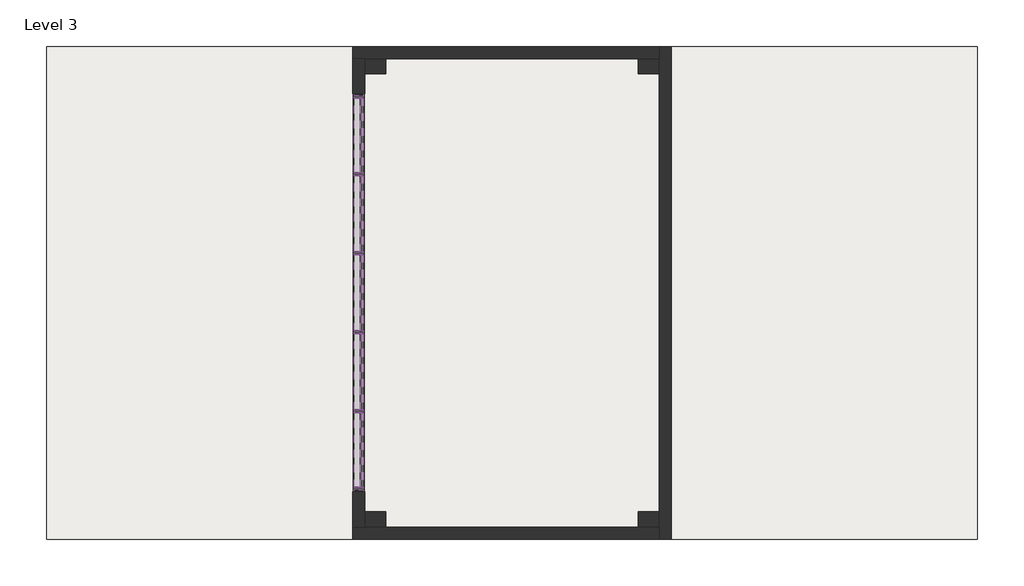
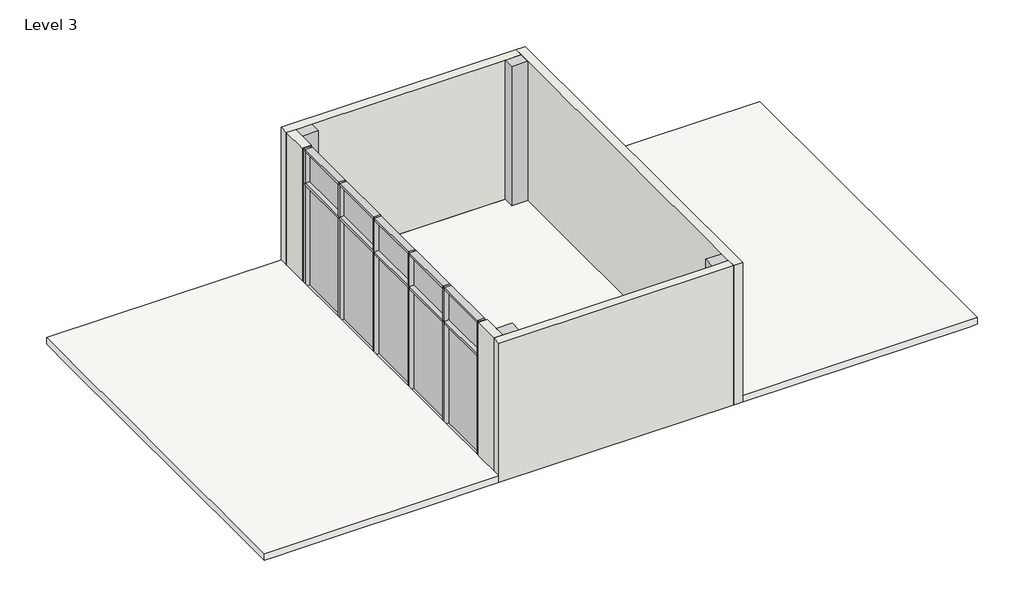
# One storey: 27 members, 10 plates, 5 walls, 4 columns, 2 roofs, 1 slab.
"""IFC4 building model written with IfcOpenShell, lengths in millimetres."""

import ifcopenshell
import ifcopenshell.guid

model = None  # the IFC model being written
_history = None  # IfcOwnerHistory: only IFC2X3 demands one
_inside = {}  # id of a spatial element -> (the spatial element, [elements in it])
_under = {}  # id of a project, library or spatial element -> (it, [spatial elements below it])
_declared = {}  # id of a project -> (the project, [libraries it declares])
_typed = {}  # id of a type object -> (the type object, [elements of that type])
_made_of = {}  # id of a material, layer set ... -> (it, [elements and type objects made of it])


def new_model(schema):
    """Start an empty IFC model of exactly this schema.

    Asked for "IFC4X3", IfcOpenShell would pick the latest addendum, in which some entities
    have other attributes; the version numbers below select the first issue.
    IFC2X3 requires an IfcOwnerHistory on every rooted entity: one is made here for all.
    """
    global model, _history
    if schema == "IFC4X3":
        model = ifcopenshell.file(schema_version=(4, 3, 0, 0))
    else:
        model = ifcopenshell.file(schema=schema)
    _inside.clear()
    _under.clear()
    _declared.clear()
    _typed.clear()
    _made_of.clear()
    _history = None
    if model.schema == "IFC2X3":
        org = make("IfcOrganization", Name="unknown")
        user = make(
            "IfcPersonAndOrganization",
            ThePerson=make("IfcPerson", FamilyName="unknown"),
            TheOrganization=org,
        )
        app = make(
            "IfcApplication",
            ApplicationDeveloper=org,
            Version="unknown",
            ApplicationFullName="unknown",
            ApplicationIdentifier="unknown",
        )
        _history = make(
            "IfcOwnerHistory",
            OwningUser=user,
            OwningApplication=app,
            ChangeAction="ADDED",
            CreationDate=0,
        )
    return model


def make(cls, **values):
    """One entity of the class cls with the attributes given. An attribute that is None is left unset."""
    return model.create_entity(
        cls, **{name: value for name, value in values.items() if value is not None}
    )


def rooted(cls, **values):
    """An entity with a GlobalId (a new one), such as an element, a storey or a relation."""
    return make(cls, GlobalId=ifcopenshell.guid.new(), OwnerHistory=_history, **values)


def si_unit(unit_type, name, prefix=None):
    """IfcSIUnit, for example si_unit("LENGTHUNIT", "METRE", prefix="MILLI")."""
    return make("IfcSIUnit", UnitType=unit_type, Prefix=prefix, Name=name)


def assignment(units):
    """IfcUnitAssignment: the units of a project."""
    return None if units is None else make("IfcUnitAssignment", Units=units)


def point(xyz):
    """IfcCartesianPoint."""
    return None if xyz is None else make("IfcCartesianPoint", Coordinates=xyz)


def direction(xyz):
    """IfcDirection."""
    return None if xyz is None else make("IfcDirection", DirectionRatios=xyz)


def frame(location, z_axis=None, x_axis=None):
    """IfcAxis2Placement3D, a coordinate frame: its origin and axes. An axis left out is left unset."""
    return make(
        "IfcAxis2Placement3D",
        Location=point(location),
        Axis=direction(z_axis),
        RefDirection=direction(x_axis),
    )


def origin():
    """The frame at (0, 0, 0) with its axes left unset."""
    return frame((0.0, 0.0, 0.0))


def origin_with_axes():
    """The frame at (0, 0, 0) with the z axis (0, 0, 1) and the x axis (1, 0, 0) written out."""
    return frame((0.0, 0.0, 0.0), z_axis=(0.0, 0.0, 1.0), x_axis=(1.0, 0.0, 0.0))


def place(relative_to, where):
    """IfcLocalPlacement: puts the frame where relative to a parent placement (None: the world)."""
    return make(
        "IfcLocalPlacement", PlacementRelTo=relative_to, RelativePlacement=where
    )


def context(
    kind, dimensions, precision=None, world=None, true_north=None, identifier=None
):
    """IfcGeometricRepresentationContext, for example the 3D "Model" context."""
    return make(
        "IfcGeometricRepresentationContext",
        ContextIdentifier=identifier,
        ContextType=kind,
        CoordinateSpaceDimension=dimensions,
        Precision=precision,
        WorldCoordinateSystem=world,
        TrueNorth=true_north,
    )


def project(units=None, contexts=None):
    """IfcProject with its units and contexts."""
    return rooted(
        "IfcProject",
        Name="project",
        RepresentationContexts=contexts,
        UnitsInContext=assignment(units),
    )


def spatial(cls, under=None, at=None, **own):
    """A site, building, storey or space (cls), placed at a placement, below another one or the project."""
    s = rooted(cls, ObjectPlacement=at, **own)
    if under is not None:
        _under.setdefault(under.id(), (under, []))[1].append(s)
    return s


def polyline(points):
    """IfcPolyline through the points."""
    return make("IfcPolyline", Points=[point(p) for p in points])


def outline(outer, holes=None, kind="AREA"):
    """IfcArbitraryClosedProfileDef: a profile drawn as a closed curve; with holes, ...WithVoids."""
    if holes is None:
        return make("IfcArbitraryClosedProfileDef", ProfileType=kind, OuterCurve=outer)
    return make(
        "IfcArbitraryProfileDefWithVoids",
        ProfileType=kind,
        OuterCurve=outer,
        InnerCurves=holes,
    )


def extrude(swept, where, along, depth):
    """IfcExtrudedAreaSolid: the profile swept, set in the frame where, extruded along a direction by depth."""
    return make(
        "IfcExtrudedAreaSolid",
        SweptArea=swept,
        Position=where,
        ExtrudedDirection=direction(along),
        Depth=depth,
    )


def faces_of(points, faces, orient=None, outer=None):
    """IfcFace entities. A face is a list of loops; a loop is a list of indices into points, from 0.

    orient and outer hold one flag for each loop. By default every Orientation is true, the
    first loop of a face is its IfcFaceOuterBound and the others are IfcFaceBound.
    """
    made = []
    for i, loops in enumerate(faces):
        bounds = []
        for j, loop in enumerate(loops):
            is_outer = j == 0 if outer is None else outer[i][j]
            bounds.append(
                make(
                    "IfcFaceOuterBound" if is_outer else "IfcFaceBound",
                    Bound=make("IfcPolyLoop", Polygon=[points[k] for k in loop]),
                    Orientation=True if orient is None else orient[i][j],
                )
            )
        made.append(make("IfcFace", Bounds=bounds))
    return made


def faceted_brep(points, faces, orient=None, outer=None, voids=None):
    """IfcFacetedBrep: a solid bounded by flat faces; with voids (closed shells), ...WithVoids."""
    shared = [point(p) for p in points]
    hull = make("IfcClosedShell", CfsFaces=faces_of(shared, faces, orient, outer))
    if voids is None:
        return make("IfcFacetedBrep", Outer=hull)
    return make(
        "IfcFacetedBrepWithVoids",
        Outer=hull,
        Voids=[
            make(cls, CfsFaces=faces_of(shared, fs, o, b)) for cls, fs, o, b in voids
        ],
    )


def shape(context_of_items, identifier, shape_type, items):
    """IfcShapeRepresentation: the items that make up one representation, for example the "Body"."""
    return make(
        "IfcShapeRepresentation",
        ContextOfItems=context_of_items,
        RepresentationIdentifier=identifier,
        RepresentationType=shape_type,
        Items=items,
    )


def source(mapping_origin, context_of_items, identifier, shape_type, items):
    """IfcRepresentationMap: a shape defined once, which mapped items show again and again."""
    return make(
        "IfcRepresentationMap",
        MappingOrigin=mapping_origin,
        MappedRepresentation=shape(context_of_items, identifier, shape_type, items),
    )


def transform(
    local_origin,
    x_axis=None,
    y_axis=None,
    z_axis=None,
    scale=None,
    scale2=None,
    scale3=None,
    uniform=True,
):
    """IfcCartesianTransformationOperator3D, or its non-uniform kind. x_axis, y_axis, z_axis: its Axis1, 2, 3."""
    if uniform:
        return make(
            "IfcCartesianTransformationOperator3D",
            Axis1=direction(x_axis),
            Axis2=direction(y_axis),
            LocalOrigin=point(local_origin),
            Scale=scale,
            Axis3=direction(z_axis),
        )
    return make(
        "IfcCartesianTransformationOperator3DnonUniform",
        Axis1=direction(x_axis),
        Axis2=direction(y_axis),
        LocalOrigin=point(local_origin),
        Scale=scale,
        Axis3=direction(z_axis),
        Scale2=scale2,
        Scale3=scale3,
    )


def mapped(mapping_source, mapping_target):
    """IfcMappedItem: shows the shape of a source again, moved by a transform."""
    return make(
        "IfcMappedItem", MappingSource=mapping_source, MappingTarget=mapping_target
    )


def made_of(thing, what):
    """Note that an element or type object is made of a material, layer set ...; save() writes the relation."""
    if what is not None:
        _made_of.setdefault(what.id(), (what, []))[1].append(thing)
    return thing


def element(
    cls,
    number,
    at=None,
    inside=None,
    cuts=None,
    type_object=None,
    material=None,
    context=None,
    identifier="Body",
    shape_type=None,
    held_by="IfcProductDefinitionShape",
    body=None,
    shapes=None,
    **own,
):
    """One element of the class cls, such as IfcWall. Its Tag is "e" and its number.

    at: its placement. inside: the storey or other place that contains it. cuts: it is an
    opening in that element (IfcRelVoidsElement). A single representation is given by context,
    identifier, shape_type and body (its items); several are given by shapes. held_by: the class
    of the entity that holds the representations. save() writes the other relations.
    """
    e = rooted(cls, Tag="e%d" % number, ObjectPlacement=at, **own)
    if body is not None:
        shapes = [shape(context, identifier, shape_type, body)]
    if shapes is not None:
        e.Representation = make(held_by, Representations=shapes)
    if inside is not None:
        _inside.setdefault(inside.id(), (inside, []))[1].append(e)
    if cuts is not None:
        rooted(
            "IfcRelVoidsElement", RelatingBuildingElement=cuts, RelatedOpeningElement=e
        )
    if type_object is not None:
        _typed.setdefault(type_object.id(), (type_object, []))[1].append(e)
    return made_of(e, material)


def aggregate(whole, parts):
    """IfcRelAggregates: a whole, such as a stair, and the parts it consists of."""
    return rooted("IfcRelAggregates", RelatingObject=whole, RelatedObjects=parts)


def save(model, path):
    """Write the relations noted so far, then the file.

    IfcRelAggregates (storeys below a building ...), IfcRelContainedInSpatialStructure (elements
    in a storey), IfcRelDefinesByType, IfcRelAssociatesMaterial and IfcRelDeclares: one each for
    every whole, place, type object, material and project.
    """
    for whole, parts in _under.values():
        aggregate(whole, parts)
    for where, things in _inside.values():
        rooted(
            "IfcRelContainedInSpatialStructure",
            RelatedElements=things,
            RelatingStructure=where,
        )
    for kind, things in _typed.values():
        rooted("IfcRelDefinesByType", RelatedObjects=things, RelatingType=kind)
    for what, things in _made_of.values():
        rooted("IfcRelAssociatesMaterial", RelatedObjects=things, RelatingMaterial=what)
    for by, libraries in _declared.values():
        rooted("IfcRelDeclares", RelatingContext=by, RelatedDefinitions=libraries)
    model.write(path)


def rectangular_mullion_50_x_150mm_49395e3f(model_context):
    return source(origin(), model_context, "Body", "SweptSolid", [
        extrude(outline(polyline([(0.0, 75.0), (0.0, -75.0), (-50.0, -75.0), (-50.0, 75.0), (0.0, 75.0)])), frame((0.0, 0.0, -1240.0000002), z_axis=(0.0, 0.0, 1.0), x_axis=(1.0, 0.0, 0.0)), (0.0, 0.0, 1.0), 1240.0000002),
    ])


def rectangular_mullion_50_x_150mm_673792d4(model_context):
    return source(origin(), model_context, "Body", "SweptSolid", [
        extrude(outline(polyline([(0.0, 75.0), (0.0, -75.0), (-50.0, -75.0), (-50.0, 75.0), (0.0, 75.0)])), frame((0.0, 0.0, -1264.9999999), z_axis=(0.0, 0.0, 1.0), x_axis=(1.0, 0.0, 0.0)), (0.0, 0.0, 1.0), 1264.9999999),
    ])


def rectangular_mullion_50_x_150mm_23e890aa(model_context):
    return source(origin(), model_context, "Body", "SweptSolid", [
        extrude(outline(polyline([(25.0, 75.0), (25.0, -75.0), (-25.0, -75.0), (-25.0, 75.0), (25.0, 75.0)])), frame((0.0, 0.0, -1240.0000002), z_axis=(0.0, 0.0, 1.0), x_axis=(1.0, 0.0, 0.0)), (0.0, 0.0, 1.0), 1240.0000002),
    ])


def rectangular_mullion_50_x_150mm_97c2790d(model_context):
    return source(origin(), model_context, "Body", "SweptSolid", [
        extrude(outline(polyline([(25.0, 75.0), (25.0, -75.0), (-25.0, -75.0), (-25.0, 75.0), (25.0, 75.0)])), frame((0.0, 0.0, -1264.9999999), z_axis=(0.0, 0.0, 1.0), x_axis=(1.0, 0.0, 0.0)), (0.0, 0.0, 1.0), 1264.9999999),
    ])


def rectangular_mullion_50_x_150mm_6225e4e3(model_context):
    return source(origin(), model_context, "Body", "SweptSolid", [
        extrude(outline(polyline([(25.0, 75.0), (25.0, -75.0), (-25.0, -75.0), (-25.0, 75.0), (25.0, 75.0)])), frame((0.0, 0.0, -2400.0), z_axis=(0.0, 0.0, 1.0), x_axis=(1.0, 0.0, 0.0)), (0.0, 0.0, 1.0), 2400.0),
    ])


def rectangular_mullion_50_x_150mm_14f10ac7(model_context):
    return source(origin(), model_context, "Body", "SweptSolid", [
        extrude(outline(polyline([(25.0, 75.0), (25.0, -75.0), (-25.0, -75.0), (-25.0, 75.0), (25.0, 75.0)])), frame((0.0, 0.0, -800.0), z_axis=(0.0, 0.0, 1.0), x_axis=(1.0, 0.0, 0.0)), (0.0, 0.0, 1.0), 800.0),
    ])


def rectangular_mullion_50_x_150mm_662c37b1(model_context):
    return source(origin(), model_context, "Body", "SweptSolid", [
        extrude(outline(polyline([(0.0, 75.0), (0.0, -75.0), (-50.0, -75.0), (-50.0, 75.0), (0.0, 75.0)])), frame((0.0, 0.0, -2400.0), z_axis=(0.0, 0.0, 1.0), x_axis=(1.0, 0.0, 0.0)), (0.0, 0.0, 1.0), 2400.0),
    ])


def rectangular_mullion_50_x_150mm_6ffebc0f(model_context):
    return source(origin(), model_context, "Body", "SweptSolid", [
        extrude(outline(polyline([(0.0, 75.0), (0.0, -75.0), (-50.0, -75.0), (-50.0, 75.0), (0.0, 75.0)])), frame((0.0, 0.0, -800.0), z_axis=(0.0, 0.0, 1.0), x_axis=(1.0, 0.0, 0.0)), (0.0, 0.0, 1.0), 800.0),
    ])


def system_panel_glazed_da598795(model_context):
    return source(origin(), model_context, "Body", "SweptSolid", [
        extrude(outline(polyline([(620.0000001, 24.5), (-620.0000001, 24.5), (-620.0000001, 49.5), (620.0000001, 49.5), (620.0000001, 24.5)])), origin_with_axes(), (0.0, 0.0, 1.0), 2325.0),
    ])


def system_panel_glazed_e4649fa4(model_context):
    return source(origin(), model_context, "Body", "SweptSolid", [
        extrude(outline(polyline([(632.4999999, 24.5), (-632.4999999, 24.5), (-632.4999999, 49.5), (632.4999999, 49.5), (632.4999999, 24.5)])), origin_with_axes(), (0.0, 0.0, 1.0), 2325.0),
    ])


def system_panel_glazed_8692f37a(model_context):
    return source(origin(), model_context, "Body", "SweptSolid", [
        extrude(outline(polyline([(620.0000001, 24.5), (-620.0000001, 24.5), (-620.0000001, 49.5), (620.0000001, 49.5), (620.0000001, 24.5)])), origin_with_axes(), (0.0, 0.0, 1.0), 725.0),
    ])


def system_panel_glazed_8e5047c4(model_context):
    return source(origin(), model_context, "Body", "SweptSolid", [
        extrude(outline(polyline([(632.4999999, 24.5), (-632.4999999, 24.5), (-632.4999999, 49.5), (632.4999999, 49.5), (632.4999999, 24.5)])), origin_with_axes(), (0.0, 0.0, 1.0), 725.0),
    ])


model = new_model("IFC4")

# Units and contexts
model_context = context("Model", 3, world=origin())
ifc_project = project(units=[si_unit("LENGTHUNIT", "METRE", prefix="MILLI")], contexts=[model_context])

# Site, building, storey
site = spatial("IfcSite", under=ifc_project)
building = spatial("IfcBuilding", under=site)
storey = spatial("IfcBuildingStorey", under=building, Name="Level 3", Elevation=6400.0)

# Columns
placement = place(None, origin())
element("IfcColumn", 1, ObjectType="M_Rectangular Column : 350 X 250", at=placement, inside=storey, context=model_context, shape_type="SweptSolid", body=[
    extrude(outline(polyline([(-376.1618676, 3056.2894154), (-26.1618676, 3056.2894154), (-26.1618676, 2806.2894154), (-376.1618676, 2806.2894154), (-376.1618676, 3056.2894154)])), frame((0.0, 0.0, 6400.0), z_axis=(0.0, 0.0, 1.0), x_axis=(1.0, 0.0, 0.0)), (0.0, 0.0, 1.0), 3200.0),
])
element("IfcColumn", 2, ObjectType="M_Rectangular Column : 350 X 250", at=placement, inside=storey, context=model_context, shape_type="SweptSolid", body=[
    extrude(outline(polyline([(-376.1618676, 10606.2894154), (-26.1618676, 10606.2894154), (-26.1618676, 10356.2894154), (-376.1618676, 10356.2894154), (-376.1618676, 10606.2894154)])), frame((0.0, 0.0, 6400.0), z_axis=(0.0, 0.0, 1.0), x_axis=(1.0, 0.0, 0.0)), (0.0, 0.0, 1.0), 3200.0),
])
element("IfcColumn", 3, ObjectType="M_Rectangular Column : 350 X 250", at=placement, inside=storey, context=model_context, shape_type="SweptSolid", body=[
    extrude(outline(polyline([(-4926.1618676, 10606.2894154), (-4576.1618676, 10606.2894154), (-4576.1618676, 10356.2894154), (-4926.1618676, 10356.2894154), (-4926.1618676, 10606.2894154)])), frame((0.0, 0.0, 6400.0), z_axis=(0.0, 0.0, 1.0), x_axis=(1.0, 0.0, 0.0)), (0.0, 0.0, 1.0), 3200.0),
])
element("IfcColumn", 4, ObjectType="M_Rectangular Column : 350 X 250", at=placement, inside=storey, context=model_context, shape_type="SweptSolid", body=[
    extrude(outline(polyline([(-4926.1618676, 3056.2894154), (-4576.1618676, 3056.2894154), (-4576.1618676, 2806.2894154), (-4926.1618676, 2806.2894154), (-4926.1618676, 3056.2894154)])), frame((0.0, 0.0, 6400.0), z_axis=(0.0, 0.0, 1.0), x_axis=(1.0, 0.0, 0.0)), (0.0, 0.0, 1.0), 3200.0),
])

# Members
rectangular_mullion_50_x_150mm_shape = rectangular_mullion_50_x_150mm_49395e3f(model_context)
element("IfcMember", 5, ObjectType="Rectangular Mullion : 50 x 150mm", at=placement, inside=storey, context=model_context, shape_type="MappedRepresentation", body=[
    mapped(rectangular_mullion_50_x_150mm_shape, transform((-5026.1618676, 3468.7894154, 9600.0), x_axis=(0.0, 0.0, 1.0), y_axis=(-1.0, 0.0, 0.0), z_axis=(0.0, -1.0, 0.0))),
])
element("IfcMember", 6, ObjectType="Rectangular Mullion : 50 x 150mm", at=placement, inside=storey, context=model_context, shape_type="MappedRepresentation", body=[
    mapped(rectangular_mullion_50_x_150mm_shape, transform((-5026.1618676, 8703.7894152, 9600.0), x_axis=(0.0, 0.0, 1.0), y_axis=(-1.0, 0.0, 0.0), z_axis=(0.0, -1.0, 0.0))),
])
element("IfcMember", 7, ObjectType="Rectangular Mullion : 50 x 150mm", at=placement, inside=storey, context=model_context, shape_type="MappedRepresentation", body=[
    mapped(rectangular_mullion_50_x_150mm_shape, transform((-5026.1618676, 9943.7894154, 6400.0), x_axis=(0.0, 0.0, -1.0), y_axis=(-1.0, 0.0, 0.0), z_axis=(0.0, 1.0, 0.0))),
])
element("IfcMember", 8, ObjectType="Rectangular Mullion : 50 x 150mm", at=placement, inside=storey, context=model_context, shape_type="MappedRepresentation", body=[
    mapped(rectangular_mullion_50_x_150mm_shape, transform((-5026.1618676, 4708.7894156, 6400.0), x_axis=(0.0, 0.0, -1.0), y_axis=(-1.0, 0.0, 0.0), z_axis=(0.0, 1.0, 0.0))),
])
rectangular_mullion_50_x_150mm_2_shape = rectangular_mullion_50_x_150mm_673792d4(model_context)
element("IfcMember", 9, ObjectType="Rectangular Mullion : 50 x 150mm", at=placement, inside=storey, context=model_context, shape_type="MappedRepresentation", body=[
    mapped(rectangular_mullion_50_x_150mm_2_shape, transform((-5026.1618676, 7388.7894153, 9600.0), x_axis=(0.0, 0.0, 1.0), y_axis=(-1.0, 0.0, 0.0), z_axis=(0.0, -1.0, 0.0))),
])
element("IfcMember", 10, ObjectType="Rectangular Mullion : 50 x 150mm", at=placement, inside=storey, context=model_context, shape_type="MappedRepresentation", body=[
    mapped(rectangular_mullion_50_x_150mm_2_shape, transform((-5026.1618676, 6073.7894154, 9600.0), x_axis=(0.0, 0.0, 1.0), y_axis=(-1.0, 0.0, 0.0), z_axis=(0.0, -1.0, 0.0))),
])
element("IfcMember", 11, ObjectType="Rectangular Mullion : 50 x 150mm", at=placement, inside=storey, context=model_context, shape_type="MappedRepresentation", body=[
    mapped(rectangular_mullion_50_x_150mm_2_shape, transform((-5026.1618676, 4758.7894156, 9600.0), x_axis=(0.0, 0.0, 1.0), y_axis=(-1.0, 0.0, 0.0), z_axis=(0.0, -1.0, 0.0))),
])
element("IfcMember", 12, ObjectType="Rectangular Mullion : 50 x 150mm", at=placement, inside=storey, context=model_context, shape_type="MappedRepresentation", body=[
    mapped(rectangular_mullion_50_x_150mm_2_shape, transform((-5026.1618676, 8653.7894152, 6400.0), x_axis=(0.0, 0.0, -1.0), y_axis=(-1.0, 0.0, 0.0), z_axis=(0.0, 1.0, 0.0))),
])
element("IfcMember", 13, ObjectType="Rectangular Mullion : 50 x 150mm", at=placement, inside=storey, context=model_context, shape_type="MappedRepresentation", body=[
    mapped(rectangular_mullion_50_x_150mm_2_shape, transform((-5026.1618676, 7338.7894153, 6400.0), x_axis=(0.0, 0.0, -1.0), y_axis=(-1.0, 0.0, 0.0), z_axis=(0.0, 1.0, 0.0))),
])
element("IfcMember", 14, ObjectType="Rectangular Mullion : 50 x 150mm", at=placement, inside=storey, context=model_context, shape_type="MappedRepresentation", body=[
    mapped(rectangular_mullion_50_x_150mm_2_shape, transform((-5026.1618676, 6023.7894154, 6400.0), x_axis=(0.0, 0.0, -1.0), y_axis=(-1.0, 0.0, 0.0), z_axis=(0.0, 1.0, 0.0))),
])
rectangular_mullion_50_x_150mm_3_shape = rectangular_mullion_50_x_150mm_23e890aa(model_context)
element("IfcMember", 15, ObjectType="Rectangular Mullion : 50 x 150mm", at=placement, inside=storey, context=model_context, shape_type="MappedRepresentation", body=[
    mapped(rectangular_mullion_50_x_150mm_3_shape, transform((-5026.1618676, 8703.7894152, 8800.0), x_axis=(0.0, 0.0, 1.0), y_axis=(-1.0, 0.0, 0.0), z_axis=(0.0, -1.0, 0.0))),
])
element("IfcMember", 16, ObjectType="Rectangular Mullion : 50 x 150mm", at=placement, inside=storey, context=model_context, shape_type="MappedRepresentation", body=[
    mapped(rectangular_mullion_50_x_150mm_3_shape, transform((-5026.1618676, 3468.7894154, 8800.0), x_axis=(0.0, 0.0, 1.0), y_axis=(-1.0, 0.0, 0.0), z_axis=(0.0, -1.0, 0.0))),
])
rectangular_mullion_50_x_150mm_4_shape = rectangular_mullion_50_x_150mm_97c2790d(model_context)
element("IfcMember", 17, ObjectType="Rectangular Mullion : 50 x 150mm", at=placement, inside=storey, context=model_context, shape_type="MappedRepresentation", body=[
    mapped(rectangular_mullion_50_x_150mm_4_shape, transform((-5026.1618676, 7388.7894153, 8800.0), x_axis=(0.0, 0.0, 1.0), y_axis=(-1.0, 0.0, 0.0), z_axis=(0.0, -1.0, 0.0))),
])
element("IfcMember", 18, ObjectType="Rectangular Mullion : 50 x 150mm", at=placement, inside=storey, context=model_context, shape_type="MappedRepresentation", body=[
    mapped(rectangular_mullion_50_x_150mm_4_shape, transform((-5026.1618676, 6073.7894154, 8800.0), x_axis=(0.0, 0.0, 1.0), y_axis=(-1.0, 0.0, 0.0), z_axis=(0.0, -1.0, 0.0))),
])
element("IfcMember", 19, ObjectType="Rectangular Mullion : 50 x 150mm", at=placement, inside=storey, context=model_context, shape_type="MappedRepresentation", body=[
    mapped(rectangular_mullion_50_x_150mm_4_shape, transform((-5026.1618676, 4758.7894156, 8800.0), x_axis=(0.0, 0.0, 1.0), y_axis=(-1.0, 0.0, 0.0), z_axis=(0.0, -1.0, 0.0))),
])
rectangular_mullion_50_x_150mm_5_shape = rectangular_mullion_50_x_150mm_6225e4e3(model_context)
element("IfcMember", 20, ObjectType="Rectangular Mullion : 50 x 150mm", at=placement, inside=storey, context=model_context, shape_type="MappedRepresentation", body=[
    mapped(rectangular_mullion_50_x_150mm_5_shape, transform((-5026.1618676, 8678.7894152, 6400.0), x_axis=(0.0, -1.0, 0.0), y_axis=(-1.0, 0.0, 0.0), z_axis=(0.0, 0.0, -1.0))),
])
element("IfcMember", 21, ObjectType="Rectangular Mullion : 50 x 150mm", at=placement, inside=storey, context=model_context, shape_type="MappedRepresentation", body=[
    mapped(rectangular_mullion_50_x_150mm_5_shape, transform((-5026.1618676, 7363.7894153, 6400.0), x_axis=(0.0, -1.0, 0.0), y_axis=(-1.0, 0.0, 0.0), z_axis=(0.0, 0.0, -1.0))),
])
element("IfcMember", 22, ObjectType="Rectangular Mullion : 50 x 150mm", at=placement, inside=storey, context=model_context, shape_type="MappedRepresentation", body=[
    mapped(rectangular_mullion_50_x_150mm_5_shape, transform((-5026.1618676, 6048.7894154, 6400.0), x_axis=(0.0, -1.0, 0.0), y_axis=(-1.0, 0.0, 0.0), z_axis=(0.0, 0.0, -1.0))),
])
element("IfcMember", 23, ObjectType="Rectangular Mullion : 50 x 150mm", at=placement, inside=storey, context=model_context, shape_type="MappedRepresentation", body=[
    mapped(rectangular_mullion_50_x_150mm_5_shape, transform((-5026.1618676, 4733.7894156, 6400.0), x_axis=(0.0, -1.0, 0.0), y_axis=(-1.0, 0.0, 0.0), z_axis=(0.0, 0.0, -1.0))),
])
rectangular_mullion_50_x_150mm_6_shape = rectangular_mullion_50_x_150mm_14f10ac7(model_context)
element("IfcMember", 24, ObjectType="Rectangular Mullion : 50 x 150mm", at=placement, inside=storey, context=model_context, shape_type="MappedRepresentation", body=[
    mapped(rectangular_mullion_50_x_150mm_6_shape, transform((-5026.1618676, 8678.7894152, 8800.0), x_axis=(0.0, -1.0, 0.0), y_axis=(-1.0, 0.0, 0.0), z_axis=(0.0, 0.0, -1.0))),
])
element("IfcMember", 25, ObjectType="Rectangular Mullion : 50 x 150mm", at=placement, inside=storey, context=model_context, shape_type="MappedRepresentation", body=[
    mapped(rectangular_mullion_50_x_150mm_6_shape, transform((-5026.1618676, 7363.7894153, 8800.0), x_axis=(0.0, -1.0, 0.0), y_axis=(-1.0, 0.0, 0.0), z_axis=(0.0, 0.0, -1.0))),
])
element("IfcMember", 26, ObjectType="Rectangular Mullion : 50 x 150mm", at=placement, inside=storey, context=model_context, shape_type="MappedRepresentation", body=[
    mapped(rectangular_mullion_50_x_150mm_6_shape, transform((-5026.1618676, 6048.7894154, 8800.0), x_axis=(0.0, -1.0, 0.0), y_axis=(-1.0, 0.0, 0.0), z_axis=(0.0, 0.0, -1.0))),
])
element("IfcMember", 27, ObjectType="Rectangular Mullion : 50 x 150mm", at=placement, inside=storey, context=model_context, shape_type="MappedRepresentation", body=[
    mapped(rectangular_mullion_50_x_150mm_6_shape, transform((-5026.1618676, 4733.7894156, 8800.0), x_axis=(0.0, -1.0, 0.0), y_axis=(-1.0, 0.0, 0.0), z_axis=(0.0, 0.0, -1.0))),
])
rectangular_mullion_50_x_150mm_7_shape = rectangular_mullion_50_x_150mm_662c37b1(model_context)
element("IfcMember", 28, ObjectType="Rectangular Mullion : 50 x 150mm", at=placement, inside=storey, context=model_context, shape_type="MappedRepresentation", body=[
    mapped(rectangular_mullion_50_x_150mm_7_shape, transform((-5026.1618676, 3418.7894154, 6400.0), x_axis=(0.0, -1.0, 0.0), y_axis=(-1.0, 0.0, 0.0), z_axis=(0.0, 0.0, -1.0))),
])
rectangular_mullion_50_x_150mm_8_shape = rectangular_mullion_50_x_150mm_6ffebc0f(model_context)
element("IfcMember", 29, ObjectType="Rectangular Mullion : 50 x 150mm", at=placement, inside=storey, context=model_context, shape_type="MappedRepresentation", body=[
    mapped(rectangular_mullion_50_x_150mm_8_shape, transform((-5026.1618676, 9993.7894154, 9600.0), x_axis=(0.0, 1.0, 0.0), y_axis=(-1.0, 0.0, 0.0), z_axis=(0.0, 0.0, 1.0))),
])
element("IfcMember", 30, ObjectType="Rectangular Mullion : 50 x 150mm", at=placement, inside=storey, context=model_context, shape_type="MappedRepresentation", body=[
    mapped(rectangular_mullion_50_x_150mm_8_shape, transform((-5026.1618676, 3418.7894154, 8800.0), x_axis=(0.0, -1.0, 0.0), y_axis=(-1.0, 0.0, 0.0), z_axis=(0.0, 0.0, -1.0))),
])
element("IfcMember", 31, ObjectType="Rectangular Mullion : 50 x 150mm", at=placement, inside=storey, context=model_context, shape_type="MappedRepresentation", body=[
    mapped(rectangular_mullion_50_x_150mm_7_shape, transform((-5026.1618676, 9993.7894154, 8800.0), x_axis=(0.0, 1.0, 0.0), y_axis=(-1.0, 0.0, 0.0), z_axis=(0.0, 0.0, 1.0))),
])

# Plates
system_panel_glazed_shape = system_panel_glazed_da598795(model_context)
element("IfcPlate", 32, ObjectType="System Panel : Glazed", at=placement, inside=storey, context=model_context, shape_type="MappedRepresentation", body=[
    mapped(system_panel_glazed_shape, transform((-5026.1618676, 9323.7894153, 6450.0), x_axis=(0.0, -1.0, 0.0), y_axis=(1.0, 0.0, 0.0), z_axis=(0.0, 0.0, 1.0))),
])
element("IfcPlate", 33, ObjectType="System Panel : Glazed", at=placement, inside=storey, context=model_context, shape_type="MappedRepresentation", body=[
    mapped(system_panel_glazed_shape, transform((-5026.1618676, 4088.7894155, 6450.0), x_axis=(0.0, -1.0, 0.0), y_axis=(1.0, 0.0, 0.0), z_axis=(0.0, 0.0, 1.0))),
])
system_panel_glazed_2_shape = system_panel_glazed_e4649fa4(model_context)
element("IfcPlate", 34, ObjectType="System Panel : Glazed", at=placement, inside=storey, context=model_context, shape_type="MappedRepresentation", body=[
    mapped(system_panel_glazed_2_shape, transform((-5026.1618676, 8021.2894153, 6450.0), x_axis=(0.0, -1.0, 0.0), y_axis=(1.0, 0.0, 0.0), z_axis=(0.0, 0.0, 1.0))),
])
element("IfcPlate", 35, ObjectType="System Panel : Glazed", at=placement, inside=storey, context=model_context, shape_type="MappedRepresentation", body=[
    mapped(system_panel_glazed_2_shape, transform((-5026.1618676, 6706.2894154, 6450.0), x_axis=(0.0, -1.0, 0.0), y_axis=(1.0, 0.0, 0.0), z_axis=(0.0, 0.0, 1.0))),
])
element("IfcPlate", 36, ObjectType="System Panel : Glazed", at=placement, inside=storey, context=model_context, shape_type="MappedRepresentation", body=[
    mapped(system_panel_glazed_2_shape, transform((-5026.1618676, 5391.2894155, 6450.0), x_axis=(0.0, -1.0, 0.0), y_axis=(1.0, 0.0, 0.0), z_axis=(0.0, 0.0, 1.0))),
])
system_panel_glazed_3_shape = system_panel_glazed_8692f37a(model_context)
element("IfcPlate", 37, ObjectType="System Panel : Glazed", at=placement, inside=storey, context=model_context, shape_type="MappedRepresentation", body=[
    mapped(system_panel_glazed_3_shape, transform((-5026.1618676, 9323.7894153, 8825.0), x_axis=(0.0, -1.0, 0.0), y_axis=(1.0, 0.0, 0.0), z_axis=(0.0, 0.0, 1.0))),
])
element("IfcPlate", 38, ObjectType="System Panel : Glazed", at=placement, inside=storey, context=model_context, shape_type="MappedRepresentation", body=[
    mapped(system_panel_glazed_3_shape, transform((-5026.1618676, 4088.7894155, 8825.0), x_axis=(0.0, -1.0, 0.0), y_axis=(1.0, 0.0, 0.0), z_axis=(0.0, 0.0, 1.0))),
])
system_panel_glazed_4_shape = system_panel_glazed_8e5047c4(model_context)
element("IfcPlate", 39, ObjectType="System Panel : Glazed", at=placement, inside=storey, context=model_context, shape_type="MappedRepresentation", body=[
    mapped(system_panel_glazed_4_shape, transform((-5026.1618676, 8021.2894153, 8825.0), x_axis=(0.0, -1.0, 0.0), y_axis=(1.0, 0.0, 0.0), z_axis=(0.0, 0.0, 1.0))),
])
element("IfcPlate", 40, ObjectType="System Panel : Glazed", at=placement, inside=storey, context=model_context, shape_type="MappedRepresentation", body=[
    mapped(system_panel_glazed_4_shape, transform((-5026.1618676, 6706.2894154, 8825.0), x_axis=(0.0, -1.0, 0.0), y_axis=(1.0, 0.0, 0.0), z_axis=(0.0, 0.0, 1.0))),
])
element("IfcPlate", 41, ObjectType="System Panel : Glazed", at=placement, inside=storey, context=model_context, shape_type="MappedRepresentation", body=[
    mapped(system_panel_glazed_4_shape, transform((-5026.1618676, 5391.2894155, 8825.0), x_axis=(0.0, -1.0, 0.0), y_axis=(1.0, 0.0, 0.0), z_axis=(0.0, 0.0, 1.0))),
])

# Roofs
element("IfcRoof", 42, ObjectType="Warm Roof - Concrete", at=placement, inside=storey, context=model_context, shape_type="Brep", body=[
    faceted_brep([(-10226.1618676, 10806.2894154, 6400.0), (-10026.1618676, 10806.2894154, 6400.0), (-5126.1618676, 10806.2894154, 6400.0), (-5126.1618676, 10606.2894154, 6400.0), (-5126.1618676, 2806.2894154, 6400.0), (-5126.1618676, 2606.2894154, 6400.0), (-6976.1618676, 2606.2894154, 6400.0), (-8013.6618676, 2606.2894154, 6400.0), (-8501.1618676, 2606.2894154, 6400.0), (-9538.6618676, 2606.2894154, 6400.0), (-10026.1618676, 2606.2894154, 6400.0), (-10226.1618676, 2606.2894154, 6400.0), (-10226.1618676, 3393.7894154, 6400.0), (-10226.1618676, 10018.7894154, 6400.0), (-5126.1618676, 10806.2894154, 6550.0), (-10226.1618676, 10806.2894154, 6550.0), (-10226.1618676, 2606.2894154, 6550.0), (-5126.1618676, 2606.2894154, 6550.0)], [[[0, 1, 2, 3, 4, 5, 6, 7, 8, 9, 10, 11, 12, 13]], [[14, 15, 16, 17]], [[15, 14, 2, 1, 0]], [[16, 15, 0, 13, 12, 11]], [[17, 16, 11, 10, 9, 8, 7, 6, 5]], [[14, 17, 5, 4, 3, 2]]]),
])
element("IfcRoof", 43, ObjectType="Warm Roof - Concrete", at=placement, inside=storey, context=model_context, shape_type="Brep", body=[
    faceted_brep([(173.8381324, 10806.2894154, 6400.0), (5073.8381324, 10806.2894154, 6400.0), (5273.8381324, 10806.2894154, 6400.0), (5273.8381324, 2606.2894154, 6400.0), (5073.8381324, 2606.2894154, 6400.0), (173.8381324, 2606.2894154, 6400.0), (5273.8381324, 10806.2894154, 6550.0), (173.8381324, 10806.2894154, 6550.0), (173.8381324, 2606.2894154, 6550.0), (5273.8381324, 2606.2894154, 6550.0)], [[[0, 1, 2, 3, 4, 5]], [[6, 7, 8, 9]], [[7, 6, 2, 1, 0]], [[8, 7, 0, 5]], [[9, 8, 5, 4, 3]], [[6, 9, 3, 2]]]),
])

# Slab
element("IfcSlab", 44, ObjectType="Standard Timber-Wood Finish", at=placement, inside=storey, context=model_context, shape_type="SweptSolid", body=[
    extrude(outline(polyline([(-26.1618676, 10606.2894154), (-26.1618676, 2806.2894154), (-4926.1618676, 2806.2894154), (-4926.1618676, 10606.2894154), (-26.1618676, 10606.2894154)])), frame((0.0, 0.0, 6350.0), z_axis=(0.0, 0.0, 1.0), x_axis=(1.0, 0.0, 0.0)), (0.0, 0.0, 1.0), 50.0),
])

# Walls
element("IfcWall", 45, ObjectType="Generic - 200mm", at=placement, inside=storey, context=model_context, shape_type="Brep", body=[
    faceted_brep([(-5126.1618676, 10606.2894154, 6400.0), (-5126.1618676, 10018.7894154, 6400.0), (-5126.1618676, 10018.7894154, 9600.0), (-5126.1618676, 10606.2894154, 9600.0), (-4926.1618676, 10606.2894154, 6400.0), (-4926.1618676, 10606.2894154, 9600.0), (-4926.1618676, 10356.2894154, 9600.0), (-4926.1618676, 10018.7894154, 9600.0), (-4926.1618676, 10018.7894154, 6400.0), (-4926.1618676, 10356.2894154, 6400.0)], [[[0, 1, 2, 3]], [[4, 5, 6, 7, 8, 9]], [[1, 0, 4, 9, 8]], [[2, 1, 8, 7]], [[3, 2, 7, 6, 5]], [[0, 3, 5, 4]]]),
])
element("IfcWall", 46, ObjectType="Generic - 200mm", at=placement, inside=storey, context=model_context, shape_type="Brep", body=[
    faceted_brep([(-26.1618676, 10806.2894154, 6400.0), (-26.1618676, 10606.2894154, 6400.0), (-26.1618676, 10356.2894154, 6400.0), (-26.1618676, 3056.2894154, 6400.0), (-26.1618676, 2806.2894154, 6400.0), (-26.1618676, 2606.2894154, 6400.0), (-26.1618676, 2606.2894154, 9600.0), (-26.1618676, 2806.2894154, 9600.0), (-26.1618676, 3056.2894154, 9600.0), (-26.1618676, 10356.2894154, 9600.0), (-26.1618676, 10606.2894154, 9600.0), (-26.1618676, 10806.2894154, 9600.0), (173.8381324, 10806.2894154, 6400.0), (173.8381324, 10806.2894154, 6550.0), (173.8381324, 10806.2894154, 9600.0), (173.8381324, 2606.2894154, 9600.0), (173.8381324, 2606.2894154, 6550.0), (173.8381324, 2606.2894154, 6400.0)], [[[0, 1, 2, 3, 4, 5, 6, 7, 8, 9, 10, 11]], [[12, 13, 14, 15, 16, 17]], [[5, 4, 3, 2, 1, 0, 12, 17]], [[11, 10, 9, 8, 7, 6, 15, 14]], [[0, 11, 14, 13, 12]], [[6, 5, 17, 16, 15]]]),
])
element("IfcWall", 47, ObjectType="Generic - 200mm", at=placement, inside=storey, context=model_context, shape_type="Brep", body=[
    faceted_brep([(-5126.1618676, 10606.2894154, 6400.0), (-4926.1618676, 10606.2894154, 6400.0), (-4576.1618676, 10606.2894154, 6400.0), (-376.1618676, 10606.2894154, 6400.0), (-26.1618676, 10606.2894154, 6400.0), (-26.1618676, 10606.2894154, 9600.0), (-376.1618676, 10606.2894154, 9600.0), (-4576.1618676, 10606.2894154, 9600.0), (-4926.1618676, 10606.2894154, 9600.0), (-5126.1618676, 10606.2894154, 9600.0), (-5126.1618676, 10806.2894154, 6400.0), (-5126.1618676, 10806.2894154, 6550.0), (-5126.1618676, 10806.2894154, 9600.0), (-26.1618676, 10806.2894154, 9600.0), (-26.1618676, 10806.2894154, 6400.0)], [[[0, 1, 2, 3, 4, 5, 6, 7, 8, 9]], [[10, 11, 12, 13, 14]], [[4, 3, 2, 1, 0, 10, 14]], [[9, 8, 7, 6, 5, 13, 12]], [[0, 9, 12, 11, 10]], [[5, 4, 14, 13]]]),
])
element("IfcWall", 48, ObjectType="Generic - 200mm", at=placement, inside=storey, context=model_context, shape_type="Brep", body=[
    faceted_brep([(-26.1618676, 2806.2894154, 6400.0), (-376.1618676, 2806.2894154, 6400.0), (-4576.1618676, 2806.2894154, 6400.0), (-4926.1618676, 2806.2894154, 6400.0), (-5126.1618676, 2806.2894154, 6400.0), (-5126.1618676, 2806.2894154, 9600.0), (-4926.1618676, 2806.2894154, 9600.0), (-4576.1618676, 2806.2894154, 9600.0), (-376.1618676, 2806.2894154, 9600.0), (-26.1618676, 2806.2894154, 9600.0), (-26.1618676, 2606.2894154, 6400.0), (-26.1618676, 2606.2894154, 9600.0), (-5126.1618676, 2606.2894154, 9600.0), (-5126.1618676, 2606.2894154, 6550.0), (-5126.1618676, 2606.2894154, 6400.0)], [[[0, 1, 2, 3, 4, 5, 6, 7, 8, 9]], [[10, 11, 12, 13, 14]], [[4, 3, 2, 1, 0, 10, 14]], [[5, 4, 14, 13, 12]], [[9, 8, 7, 6, 5, 12, 11]], [[0, 9, 11, 10]]]),
])
element("IfcWall", 49, ObjectType="Generic - 200mm", at=placement, inside=storey, context=model_context, shape_type="Brep", body=[
    faceted_brep([(-5126.1618676, 3393.7894154, 6400.0), (-5126.1618676, 2806.2894154, 6400.0), (-5126.1618676, 2806.2894154, 9600.0), (-5126.1618676, 3393.7894154, 9600.0), (-4926.1618676, 3393.7894154, 6400.0), (-4926.1618676, 3393.7894154, 9600.0), (-4926.1618676, 3056.2894154, 9600.0), (-4926.1618676, 2806.2894154, 9600.0), (-4926.1618676, 2806.2894154, 6400.0), (-4926.1618676, 3056.2894154, 6400.0)], [[[0, 1, 2, 3]], [[4, 5, 6, 7, 8, 9]], [[1, 0, 4, 9, 8]], [[3, 2, 7, 6, 5]], [[0, 3, 5, 4]], [[2, 1, 8, 7]]]),
])

save(model, "model.ifc")

# Revit data of these elements
# Type "M_Rectangular Column : 350 X 250"
#   Depth = 0.35 m
#   Offset Base = 0.00 m
#   Offset Top = 0.00 m
#   Width = 0.25 m
#   Material = none
# Type "Rectangular Mullion : 50 x 150mm"
#   built-in parameter 1007304 = 0.492126 (stored number, unit not read)
#   built-in parameter 1007301 = 0.082021 (stored number, unit not read)
#   built-in parameter 1007300 = 0.082021 (stored number, unit not read)
# Type "System Panel : Glazed"
#   Construction Type Id = "GSP4R"
#   Analytic Construction = "1/8 in Pilkington single glazing"
#   Visual Light Transmittance = 0.9
#   Solar Heat Gain Coefficient = 0.86
#   Heat Transfer Coefficient (U) = 6.7069 W/(m²·K)
#   Define Thermal Properties by = 1
# Type "Warm Roof - Concrete"
#   Layers, outside or top first: 0.02 m "Concrete, Cast In Situ" (function 4); 0.05 m "Rigid insulation" (function 3); 0.02 m "Asphalt, Bitumen" (function 3); 0.00 m "Roofing Felt" (function 100); 0.05 m "Concrete, Sand/Cement Screed" (function 2); 0.01 m "Concrete, Cast In Situ" (function 1)
# Type "Standard Timber-Wood Finish"
#   Function = 0
#   Layers, outside or top first: 0.03 m "Oak Flooring" (function 5); 0.02 m "Wood Sheathing, Chipboard" (function 1)
# Type "Generic - 200mm"
#   Layers, outside or top first: 0.20 m "Concrete, Cast In Situ" (function 1)
# Elements 1, 2, 3, 4 (IfcColumn, "M_Rectangular Column : 350 X 250")
#   Phase Created = New Construction
#   Materials on its faces: "Concrete, Cast In Situ"
# Elements 5, 6, 7, 8, 9, 10, 11, 12, 13, 14, 15, 16, 17, 18, 19, 20, 21, 22, 23, 24, 25, 26, 27, 28, 29, 30, 31 (IfcMember, "Rectangular Mullion : 50 x 150mm")
#   Phase Created = New Construction
#   Materials on its faces: "Aluminium"
# Elements 32, 33, 34, 35, 36, 37, 38, 39, 40, 41 (IfcPlate, "System Panel : Glazed")
#   Phase Created = New Construction
#   Materials on its faces: "Glass"
# Elements 42, 43 (IfcRoof, "Warm Roof - Concrete")
#   built-in parameter 1001705 = 21.4895 (stored number, unit not read)
#   built-in parameter 1001710 = 33615
#   Phase Created = New Construction
#   Materials on its faces: "Concrete, Cast In Situ"
# Element 44 (IfcSlab, "Standard Timber-Wood Finish")
#   Height Offset From Level = 0.00 m
#   Phase Created = New Construction
#   Materials on its faces: "Wood Sheathing, Chipboard", "Oak Flooring"
# Elements 45, 46, 47, 48, 49 (IfcWall, "Generic - 200mm")
#   Top Offset = 0.00 m
#   Base Offset = 0.00 m
#   wall height = 3.20 m
#   Phase Created = New Construction
#   Base Constraint = Level 3
#   Top Constraint = Level 4
#   Materials on its faces: "Concrete, Cast In Situ"
# Materials
#   "Concrete, Cast In Situ": class "Concrete", colour RGB 192 192 192, transparency 0, Description = "physical material", Cost = 0
#   "Rigid insulation": class "Generic", colour RGB 127 127 127, transparency 0, Description = "Rigid foam insulation board", Cost = 0
#   "Asphalt, Bitumen": class "Generic", colour RGB 155 155 155, transparency 0, Description = "Bituminous roofing material", Cost = 0
#   "Roofing Felt": class "Generic", colour RGB 127 127 127, transparency 0, Description = "Asphalt saturated felt", Cost = 0
#   "Concrete, Sand/Cement Screed": class "Concrete", colour RGB 127 127 127, transparency 0, Description = "Concrete slab topping", Cost = 0
#   "Oak Flooring": class "Wood", colour RGB 212 179 113, transparency 0, Description = "Quercus Rubra", Cost = 0
#   "Wood Sheathing, Chipboard": class "Wood", colour RGB 108 95 74, transparency 0, Description = "Particleboard sheathing", Cost = 0
#   "Aluminium": class "Metal", colour RGB 247 247 247, transparency 0, Description = "Aluminium 6061", Cost = 0
#   "Glass": class "Glass", colour RGB 0 128 192, transparency 0.9, Description = "Soda Lime Glass", Cost = 0
